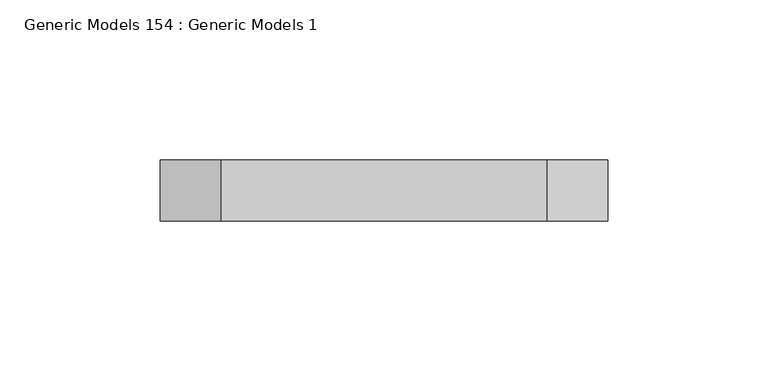
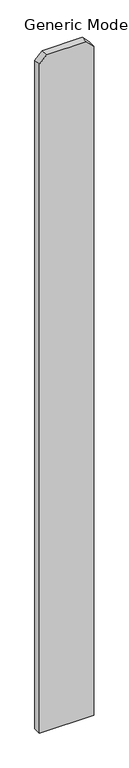
"""IFC4 building model written with IfcOpenShell, lengths in millimetres: proxy geometry, Generic Models 154 : Generic Models 1."""

import ifcopenshell
import ifcopenshell.guid

model = None  # the IFC model being written
_history = None  # IfcOwnerHistory: only IFC2X3 demands one
_inside = {}  # id of a spatial element -> (the spatial element, [elements in it])
_under = {}  # id of a project, library or spatial element -> (it, [spatial elements below it])
_declared = {}  # id of a project -> (the project, [libraries it declares])
_typed = {}  # id of a type object -> (the type object, [elements of that type])
_made_of = {}  # id of a material, layer set ... -> (it, [elements and type objects made of it])


def new_model(schema):
    """Start an empty IFC model of exactly this schema.

    Asked for "IFC4X3", IfcOpenShell would pick the latest addendum, in which some entities
    have other attributes; the version numbers below select the first issue.
    IFC2X3 requires an IfcOwnerHistory on every rooted entity: one is made here for all.
    """
    global model, _history
    if schema == "IFC4X3":
        model = ifcopenshell.file(schema_version=(4, 3, 0, 0))
    else:
        model = ifcopenshell.file(schema=schema)
    _inside.clear()
    _under.clear()
    _declared.clear()
    _typed.clear()
    _made_of.clear()
    _history = None
    if model.schema == "IFC2X3":
        org = make("IfcOrganization", Name="unknown")
        user = make(
            "IfcPersonAndOrganization",
            ThePerson=make("IfcPerson", FamilyName="unknown"),
            TheOrganization=org,
        )
        app = make(
            "IfcApplication",
            ApplicationDeveloper=org,
            Version="unknown",
            ApplicationFullName="unknown",
            ApplicationIdentifier="unknown",
        )
        _history = make(
            "IfcOwnerHistory",
            OwningUser=user,
            OwningApplication=app,
            ChangeAction="ADDED",
            CreationDate=0,
        )
    return model


def make(cls, **values):
    """One entity of the class cls with the attributes given. An attribute that is None is left unset."""
    return model.create_entity(
        cls, **{name: value for name, value in values.items() if value is not None}
    )


def rooted(cls, **values):
    """An entity with a GlobalId (a new one), such as an element, a storey or a relation."""
    return make(cls, GlobalId=ifcopenshell.guid.new(), OwnerHistory=_history, **values)


def si_unit(unit_type, name, prefix=None):
    """IfcSIUnit, for example si_unit("LENGTHUNIT", "METRE", prefix="MILLI")."""
    return make("IfcSIUnit", UnitType=unit_type, Prefix=prefix, Name=name)


def assignment(units):
    """IfcUnitAssignment: the units of a project."""
    return None if units is None else make("IfcUnitAssignment", Units=units)


def point(xyz):
    """IfcCartesianPoint."""
    return None if xyz is None else make("IfcCartesianPoint", Coordinates=xyz)


def direction(xyz):
    """IfcDirection."""
    return None if xyz is None else make("IfcDirection", DirectionRatios=xyz)


def frame(location, z_axis=None, x_axis=None):
    """IfcAxis2Placement3D, a coordinate frame: its origin and axes. An axis left out is left unset."""
    return make(
        "IfcAxis2Placement3D",
        Location=point(location),
        Axis=direction(z_axis),
        RefDirection=direction(x_axis),
    )


def origin():
    """The frame at (0, 0, 0) with its axes left unset."""
    return frame((0.0, 0.0, 0.0))


def place(relative_to, where):
    """IfcLocalPlacement: puts the frame where relative to a parent placement (None: the world)."""
    return make(
        "IfcLocalPlacement", PlacementRelTo=relative_to, RelativePlacement=where
    )


def context(
    kind, dimensions, precision=None, world=None, true_north=None, identifier=None
):
    """IfcGeometricRepresentationContext, for example the 3D "Model" context."""
    return make(
        "IfcGeometricRepresentationContext",
        ContextIdentifier=identifier,
        ContextType=kind,
        CoordinateSpaceDimension=dimensions,
        Precision=precision,
        WorldCoordinateSystem=world,
        TrueNorth=true_north,
    )


def project(units=None, contexts=None):
    """IfcProject with its units and contexts."""
    return rooted(
        "IfcProject",
        Name="project",
        RepresentationContexts=contexts,
        UnitsInContext=assignment(units),
    )


def spatial(cls, under=None, at=None, **own):
    """A site, building, storey or space (cls), placed at a placement, below another one or the project."""
    s = rooted(cls, ObjectPlacement=at, **own)
    if under is not None:
        _under.setdefault(under.id(), (under, []))[1].append(s)
    return s


def polyline(points):
    """IfcPolyline through the points."""
    return make("IfcPolyline", Points=[point(p) for p in points])


def outline(outer, holes=None, kind="AREA"):
    """IfcArbitraryClosedProfileDef: a profile drawn as a closed curve; with holes, ...WithVoids."""
    if holes is None:
        return make("IfcArbitraryClosedProfileDef", ProfileType=kind, OuterCurve=outer)
    return make(
        "IfcArbitraryProfileDefWithVoids",
        ProfileType=kind,
        OuterCurve=outer,
        InnerCurves=holes,
    )


def extrude(swept, where, along, depth):
    """IfcExtrudedAreaSolid: the profile swept, set in the frame where, extruded along a direction by depth."""
    return make(
        "IfcExtrudedAreaSolid",
        SweptArea=swept,
        Position=where,
        ExtrudedDirection=direction(along),
        Depth=depth,
    )


def shape(context_of_items, identifier, shape_type, items):
    """IfcShapeRepresentation: the items that make up one representation, for example the "Body"."""
    return make(
        "IfcShapeRepresentation",
        ContextOfItems=context_of_items,
        RepresentationIdentifier=identifier,
        RepresentationType=shape_type,
        Items=items,
    )


def source(mapping_origin, context_of_items, identifier, shape_type, items):
    """IfcRepresentationMap: a shape defined once, which mapped items show again and again."""
    return make(
        "IfcRepresentationMap",
        MappingOrigin=mapping_origin,
        MappedRepresentation=shape(context_of_items, identifier, shape_type, items),
    )


def transform(
    local_origin,
    x_axis=None,
    y_axis=None,
    z_axis=None,
    scale=None,
    scale2=None,
    scale3=None,
    uniform=True,
):
    """IfcCartesianTransformationOperator3D, or its non-uniform kind. x_axis, y_axis, z_axis: its Axis1, 2, 3."""
    if uniform:
        return make(
            "IfcCartesianTransformationOperator3D",
            Axis1=direction(x_axis),
            Axis2=direction(y_axis),
            LocalOrigin=point(local_origin),
            Scale=scale,
            Axis3=direction(z_axis),
        )
    return make(
        "IfcCartesianTransformationOperator3DnonUniform",
        Axis1=direction(x_axis),
        Axis2=direction(y_axis),
        LocalOrigin=point(local_origin),
        Scale=scale,
        Axis3=direction(z_axis),
        Scale2=scale2,
        Scale3=scale3,
    )


def mapped(mapping_source, mapping_target):
    """IfcMappedItem: shows the shape of a source again, moved by a transform."""
    return make(
        "IfcMappedItem", MappingSource=mapping_source, MappingTarget=mapping_target
    )


def made_of(thing, what):
    """Note that an element or type object is made of a material, layer set ...; save() writes the relation."""
    if what is not None:
        _made_of.setdefault(what.id(), (what, []))[1].append(thing)
    return thing


def element(
    cls,
    number,
    at=None,
    inside=None,
    cuts=None,
    type_object=None,
    material=None,
    context=None,
    identifier="Body",
    shape_type=None,
    held_by="IfcProductDefinitionShape",
    body=None,
    shapes=None,
    **own,
):
    """One element of the class cls, such as IfcWall. Its Tag is "e" and its number.

    at: its placement. inside: the storey or other place that contains it. cuts: it is an
    opening in that element (IfcRelVoidsElement). A single representation is given by context,
    identifier, shape_type and body (its items); several are given by shapes. held_by: the class
    of the entity that holds the representations. save() writes the other relations.
    """
    e = rooted(cls, Tag="e%d" % number, ObjectPlacement=at, **own)
    if body is not None:
        shapes = [shape(context, identifier, shape_type, body)]
    if shapes is not None:
        e.Representation = make(held_by, Representations=shapes)
    if inside is not None:
        _inside.setdefault(inside.id(), (inside, []))[1].append(e)
    if cuts is not None:
        rooted(
            "IfcRelVoidsElement", RelatingBuildingElement=cuts, RelatedOpeningElement=e
        )
    if type_object is not None:
        _typed.setdefault(type_object.id(), (type_object, []))[1].append(e)
    return made_of(e, material)


def aggregate(whole, parts):
    """IfcRelAggregates: a whole, such as a stair, and the parts it consists of."""
    return rooted("IfcRelAggregates", RelatingObject=whole, RelatedObjects=parts)


def save(model, path):
    """Write the relations noted so far, then the file.

    IfcRelAggregates (storeys below a building ...), IfcRelContainedInSpatialStructure (elements
    in a storey), IfcRelDefinesByType, IfcRelAssociatesMaterial and IfcRelDeclares: one each for
    every whole, place, type object, material and project.
    """
    for whole, parts in _under.values():
        aggregate(whole, parts)
    for where, things in _inside.values():
        rooted(
            "IfcRelContainedInSpatialStructure",
            RelatedElements=things,
            RelatingStructure=where,
        )
    for kind, things in _typed.values():
        rooted("IfcRelDefinesByType", RelatedObjects=things, RelatingType=kind)
    for what, things in _made_of.values():
        rooted("IfcRelAssociatesMaterial", RelatedObjects=things, RelatingMaterial=what)
    for by, libraries in _declared.values():
        rooted("IfcRelDeclares", RelatingContext=by, RelatedDefinitions=libraries)
    model.write(path)


def generic_models_154_generic_models_1_06d36a19(model_context):
    return source(origin(), model_context, "Body", "SweptSolid", [
        extrude(outline(polyline([(76.2, 53922.6125), (1885.95, 53922.6125), (1905.0, 53903.5625), (1905.0, 53801.9625), (1885.95, 53782.9125), (76.2, 53782.9125), (76.2, 53922.6125)])), frame((0.0, 547.6875, 0.0), z_axis=(0.0, 1.0, 0.0), x_axis=(0.0, 0.0, 1.0)), (0.0, 0.0, 1.0), 19.05),
    ])


if __name__ == "__main__":
    model = new_model("IFC4")
    model_context = context("Model", 3, world=origin())
    ifc_project = project(units=[si_unit("LENGTHUNIT", "METRE", prefix="MILLI")], contexts=[model_context])
    site = spatial("IfcSite", under=ifc_project)
    building = spatial("IfcBuilding", under=site)
    placement = place(None, origin())
    generic_models_154_generic_models_1_shape = generic_models_154_generic_models_1_06d36a19(model_context)
    element("IfcBuildingElementProxy", 1, Name="Generic Models 154 : Generic Models 1", ObjectType="Generic Models 154 : Generic Models 1", at=placement, inside=building, context=model_context, shape_type="MappedRepresentation", body=[
        mapped(generic_models_154_generic_models_1_shape, transform((0.0, 0.0, 0.0), x_axis=(1.0, 0.0, 0.0), y_axis=(0.0, 1.0, 0.0), z_axis=(0.0, 0.0, 1.0))),
    ])
    save(model, "model.ifc")

# Revit data of these elements
# Element 1 (IfcBuildingElementProxy, "Generic Models 154 : Generic Models 1")
#   Materials on its faces: "VERTICAL 1X6 CEDAR PLANKS W/ CLEAR WOOD SEALER"
# Materials
#   "VERTICAL 1X6 CEDAR PLANKS W/ CLEAR WOOD SEALER": class "Wood", colour RGB 234 198 147, transparency 0, Description = "Pinus Echinata", Cost = 0
